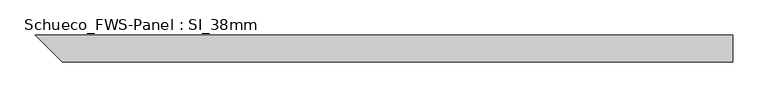
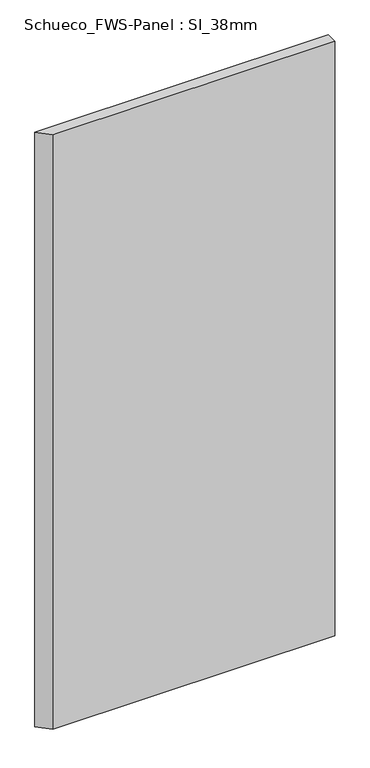
"""IFC4 building model written with IfcOpenShell, lengths in millimetres: plate geometry, Schueco_FWS-Panel : SI_38mm."""

from ifc_helpers import new_model, si_unit, origin, origin_with_axes, place, context, project, spatial, polyline, outline, extrude, source, transform, mapped, element, save


def schueco_fws_panel_si_38mm_18656d05(model_context):
    return source(origin(), model_context, "Body", "SweptSolid", [
        extrude(outline(polyline([(-492.0, 0.0), (492.0, 0.0), (492.0, -38.0), (-454.0, -38.0), (-492.0, 0.0)])), origin_with_axes(), (0.0, 0.0, 1.0), 2108.0),
    ])


if __name__ == "__main__":
    model = new_model("IFC4")
    model_context = context("Model", 3, world=origin())
    ifc_project = project(units=[si_unit("LENGTHUNIT", "METRE", prefix="MILLI")], contexts=[model_context])
    site = spatial("IfcSite", under=ifc_project)
    building = spatial("IfcBuilding", under=site)
    placement = place(None, origin())
    schueco_fws_panel_si_38mm_shape = schueco_fws_panel_si_38mm_18656d05(model_context)
    element("IfcPlate", 1, ObjectType="Schueco_FWS-Panel : SI_38mm", at=placement, inside=building, context=model_context, shape_type="MappedRepresentation", body=[
        mapped(schueco_fws_panel_si_38mm_shape, transform((0.0, 0.0, 0.0), x_axis=(1.0, 0.0, 0.0), y_axis=(0.0, 1.0, 0.0), z_axis=(0.0, 0.0, 1.0))),
    ])
    save(model, "model.ifc")

# Revit data of these elements
# Type "Schueco_FWS-Panel : SI_38mm"
#   Model = "Panel 38mm"
#   Manufacturer = "Schueco International KG"
#   Analytic Construction = "<Keine Auswahl>"
#   Panel thickness = 38 mm
#   Angle right [instance default] = 0.00°
#   Angle left [instance default] = 0.00°
#   AR [instance default] = 0.00°
#   AL [instance default] = 0.00°
#   FWS SI insert unit = yes
#   FWS HI insert unit = no
#   Det_R [instance default] = yes
#   Det_L [instance default] = yes
#   Panel = Alu
# Element 1 (IfcPlate, "Schueco_FWS-Panel : SI_38mm")
#   Angle left = 45.00°
#   AL = 45.00°
#   Det_L = no
#   Materials on its faces: "Alu"
# Materials
#   "Alu": class "Glas", colour RGB 140 140 140, transparency 0
